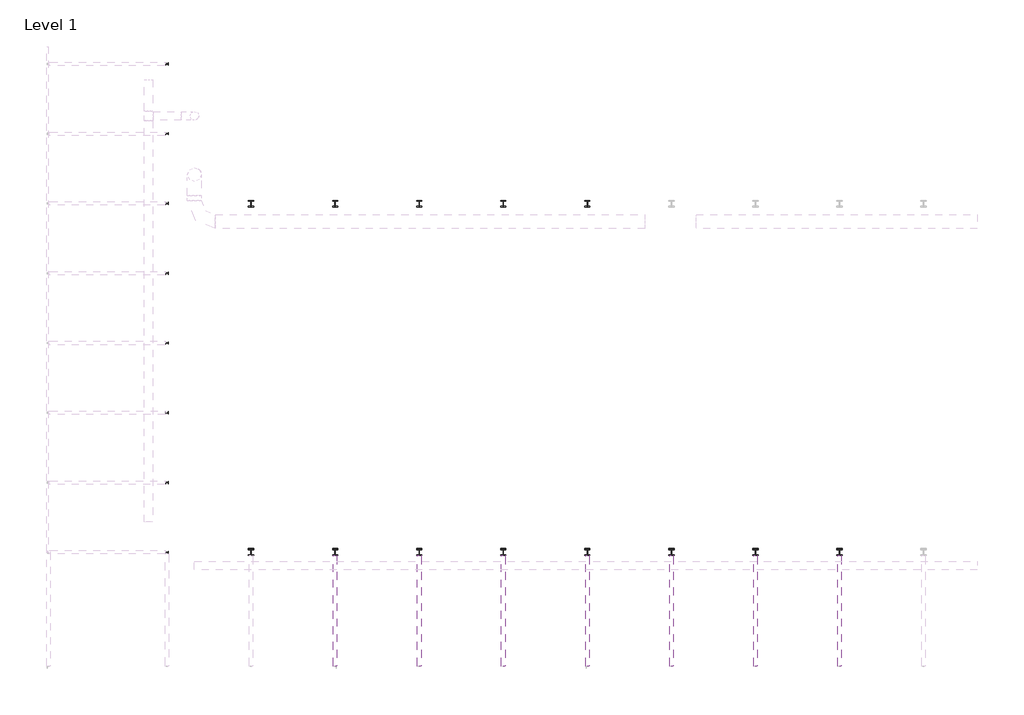
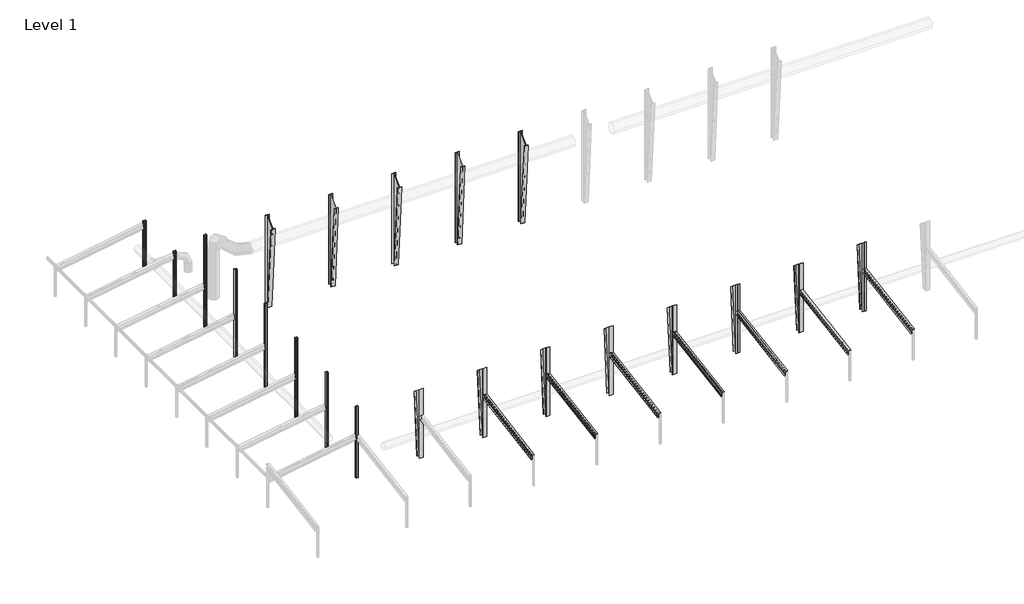
# One storey, part 2 of 3: 21 columns, 7 beams.
"""IFC4 building model written with IfcOpenShell, lengths in millimetres."""

import ifcopenshell
import ifcopenshell.guid

model = None  # the IFC model being written
_history = None  # IfcOwnerHistory: only IFC2X3 demands one
_inside = {}  # id of a spatial element -> (the spatial element, [elements in it])
_under = {}  # id of a project, library or spatial element -> (it, [spatial elements below it])
_declared = {}  # id of a project -> (the project, [libraries it declares])
_typed = {}  # id of a type object -> (the type object, [elements of that type])
_made_of = {}  # id of a material, layer set ... -> (it, [elements and type objects made of it])


def new_model(schema):
    """Start an empty IFC model of exactly this schema.

    Asked for "IFC4X3", IfcOpenShell would pick the latest addendum, in which some entities
    have other attributes; the version numbers below select the first issue.
    IFC2X3 requires an IfcOwnerHistory on every rooted entity: one is made here for all.
    """
    global model, _history
    if schema == "IFC4X3":
        model = ifcopenshell.file(schema_version=(4, 3, 0, 0))
    else:
        model = ifcopenshell.file(schema=schema)
    _inside.clear()
    _under.clear()
    _declared.clear()
    _typed.clear()
    _made_of.clear()
    _history = None
    if model.schema == "IFC2X3":
        org = make("IfcOrganization", Name="unknown")
        user = make(
            "IfcPersonAndOrganization",
            ThePerson=make("IfcPerson", FamilyName="unknown"),
            TheOrganization=org,
        )
        app = make(
            "IfcApplication",
            ApplicationDeveloper=org,
            Version="unknown",
            ApplicationFullName="unknown",
            ApplicationIdentifier="unknown",
        )
        _history = make(
            "IfcOwnerHistory",
            OwningUser=user,
            OwningApplication=app,
            ChangeAction="ADDED",
            CreationDate=0,
        )
    return model


def make(cls, **values):
    """One entity of the class cls with the attributes given. An attribute that is None is left unset."""
    return model.create_entity(
        cls, **{name: value for name, value in values.items() if value is not None}
    )


def rooted(cls, **values):
    """An entity with a GlobalId (a new one), such as an element, a storey or a relation."""
    return make(cls, GlobalId=ifcopenshell.guid.new(), OwnerHistory=_history, **values)


def si_unit(unit_type, name, prefix=None):
    """IfcSIUnit, for example si_unit("LENGTHUNIT", "METRE", prefix="MILLI")."""
    return make("IfcSIUnit", UnitType=unit_type, Prefix=prefix, Name=name)


def assignment(units):
    """IfcUnitAssignment: the units of a project."""
    return None if units is None else make("IfcUnitAssignment", Units=units)


def point(xyz):
    """IfcCartesianPoint."""
    return None if xyz is None else make("IfcCartesianPoint", Coordinates=xyz)


def direction(xyz):
    """IfcDirection."""
    return None if xyz is None else make("IfcDirection", DirectionRatios=xyz)


def frame(location, z_axis=None, x_axis=None):
    """IfcAxis2Placement3D, a coordinate frame: its origin and axes. An axis left out is left unset."""
    return make(
        "IfcAxis2Placement3D",
        Location=point(location),
        Axis=direction(z_axis),
        RefDirection=direction(x_axis),
    )


def frame_2d(location, x_axis=None):
    """IfcAxis2Placement2D, a coordinate frame in the plane: its origin and x axis."""
    return make(
        "IfcAxis2Placement2D", Location=point(location), RefDirection=direction(x_axis)
    )


def origin():
    """The frame at (0, 0, 0) with its axes left unset."""
    return frame((0.0, 0.0, 0.0))


def origin_with_axes():
    """The frame at (0, 0, 0) with the z axis (0, 0, 1) and the x axis (1, 0, 0) written out."""
    return frame((0.0, 0.0, 0.0), z_axis=(0.0, 0.0, 1.0), x_axis=(1.0, 0.0, 0.0))


def place(relative_to, where):
    """IfcLocalPlacement: puts the frame where relative to a parent placement (None: the world)."""
    return make(
        "IfcLocalPlacement", PlacementRelTo=relative_to, RelativePlacement=where
    )


def context(
    kind, dimensions, precision=None, world=None, true_north=None, identifier=None
):
    """IfcGeometricRepresentationContext, for example the 3D "Model" context."""
    return make(
        "IfcGeometricRepresentationContext",
        ContextIdentifier=identifier,
        ContextType=kind,
        CoordinateSpaceDimension=dimensions,
        Precision=precision,
        WorldCoordinateSystem=world,
        TrueNorth=true_north,
    )


def project(units=None, contexts=None):
    """IfcProject with its units and contexts."""
    return rooted(
        "IfcProject",
        Name="project",
        RepresentationContexts=contexts,
        UnitsInContext=assignment(units),
    )


def spatial(cls, under=None, at=None, **own):
    """A site, building, storey or space (cls), placed at a placement, below another one or the project."""
    s = rooted(cls, ObjectPlacement=at, **own)
    if under is not None:
        _under.setdefault(under.id(), (under, []))[1].append(s)
    return s


def polyline(points):
    """IfcPolyline through the points."""
    return make("IfcPolyline", Points=[point(p) for p in points])


def circle_curve(where, radius):
    """IfcCircle in the frame where."""
    return make("IfcCircle", Position=where, Radius=radius)


def trimmed(basis, trim1, trim2, sense, master):
    """IfcTrimmedCurve: the piece of a basis curve between two trims."""
    return make(
        "IfcTrimmedCurve",
        BasisCurve=basis,
        Trim1=trim1,
        Trim2=trim2,
        SenseAgreement=sense,
        MasterRepresentation=master,
    )


def segment(curve, same_sense, transition):
    """IfcCompositeCurveSegment."""
    return make(
        "IfcCompositeCurveSegment",
        Transition=transition,
        SameSense=same_sense,
        ParentCurve=curve,
    )


def composite_curve(segments, self_intersect=None):
    """IfcCompositeCurve: segments joined end to end."""
    return make("IfcCompositeCurve", Segments=segments, SelfIntersect=self_intersect)


def outline(outer, holes=None, kind="AREA"):
    """IfcArbitraryClosedProfileDef: a profile drawn as a closed curve; with holes, ...WithVoids."""
    if holes is None:
        return make("IfcArbitraryClosedProfileDef", ProfileType=kind, OuterCurve=outer)
    return make(
        "IfcArbitraryProfileDefWithVoids",
        ProfileType=kind,
        OuterCurve=outer,
        InnerCurves=holes,
    )


def extrude(swept, where, along, depth):
    """IfcExtrudedAreaSolid: the profile swept, set in the frame where, extruded along a direction by depth."""
    return make(
        "IfcExtrudedAreaSolid",
        SweptArea=swept,
        Position=where,
        ExtrudedDirection=direction(along),
        Depth=depth,
    )


def shape(context_of_items, identifier, shape_type, items):
    """IfcShapeRepresentation: the items that make up one representation, for example the "Body"."""
    return make(
        "IfcShapeRepresentation",
        ContextOfItems=context_of_items,
        RepresentationIdentifier=identifier,
        RepresentationType=shape_type,
        Items=items,
    )


def source(mapping_origin, context_of_items, identifier, shape_type, items):
    """IfcRepresentationMap: a shape defined once, which mapped items show again and again."""
    return make(
        "IfcRepresentationMap",
        MappingOrigin=mapping_origin,
        MappedRepresentation=shape(context_of_items, identifier, shape_type, items),
    )


def transform(
    local_origin,
    x_axis=None,
    y_axis=None,
    z_axis=None,
    scale=None,
    scale2=None,
    scale3=None,
    uniform=True,
):
    """IfcCartesianTransformationOperator3D, or its non-uniform kind. x_axis, y_axis, z_axis: its Axis1, 2, 3."""
    if uniform:
        return make(
            "IfcCartesianTransformationOperator3D",
            Axis1=direction(x_axis),
            Axis2=direction(y_axis),
            LocalOrigin=point(local_origin),
            Scale=scale,
            Axis3=direction(z_axis),
        )
    return make(
        "IfcCartesianTransformationOperator3DnonUniform",
        Axis1=direction(x_axis),
        Axis2=direction(y_axis),
        LocalOrigin=point(local_origin),
        Scale=scale,
        Axis3=direction(z_axis),
        Scale2=scale2,
        Scale3=scale3,
    )


def mapped(mapping_source, mapping_target):
    """IfcMappedItem: shows the shape of a source again, moved by a transform."""
    return make(
        "IfcMappedItem", MappingSource=mapping_source, MappingTarget=mapping_target
    )


def made_of(thing, what):
    """Note that an element or type object is made of a material, layer set ...; save() writes the relation."""
    if what is not None:
        _made_of.setdefault(what.id(), (what, []))[1].append(thing)
    return thing


def element(
    cls,
    number,
    at=None,
    inside=None,
    cuts=None,
    type_object=None,
    material=None,
    context=None,
    identifier="Body",
    shape_type=None,
    held_by="IfcProductDefinitionShape",
    body=None,
    shapes=None,
    **own,
):
    """One element of the class cls, such as IfcWall. Its Tag is "e" and its number.

    at: its placement. inside: the storey or other place that contains it. cuts: it is an
    opening in that element (IfcRelVoidsElement). A single representation is given by context,
    identifier, shape_type and body (its items); several are given by shapes. held_by: the class
    of the entity that holds the representations. save() writes the other relations.
    """
    e = rooted(cls, Tag="e%d" % number, ObjectPlacement=at, **own)
    if body is not None:
        shapes = [shape(context, identifier, shape_type, body)]
    if shapes is not None:
        e.Representation = make(held_by, Representations=shapes)
    if inside is not None:
        _inside.setdefault(inside.id(), (inside, []))[1].append(e)
    if cuts is not None:
        rooted(
            "IfcRelVoidsElement", RelatingBuildingElement=cuts, RelatedOpeningElement=e
        )
    if type_object is not None:
        _typed.setdefault(type_object.id(), (type_object, []))[1].append(e)
    return made_of(e, material)


def aggregate(whole, parts):
    """IfcRelAggregates: a whole, such as a stair, and the parts it consists of."""
    return rooted("IfcRelAggregates", RelatingObject=whole, RelatedObjects=parts)


def save(model, path):
    """Write the relations noted so far, then the file.

    IfcRelAggregates (storeys below a building ...), IfcRelContainedInSpatialStructure (elements
    in a storey), IfcRelDefinesByType, IfcRelAssociatesMaterial and IfcRelDeclares: one each for
    every whole, place, type object, material and project.
    """
    for whole, parts in _under.values():
        aggregate(whole, parts)
    for where, things in _inside.values():
        rooted(
            "IfcRelContainedInSpatialStructure",
            RelatedElements=things,
            RelatingStructure=where,
        )
    for kind, things in _typed.values():
        rooted("IfcRelDefinesByType", RelatedObjects=things, RelatingType=kind)
    for what, things in _made_of.values():
        rooted("IfcRelAssociatesMaterial", RelatedObjects=things, RelatingMaterial=what)
    for by, libraries in _declared.values():
        rooted("IfcRelDeclares", RelatingContext=by, RelatedDefinitions=libraries)
    model.write(path)


def w_wide_flange_w21x166_c1e76bd8(model_context):
    return source(origin(), model_context, "Body", "SweptSolid", [
        extrude(outline(composite_curve([segment(polyline([(157.48, -251.206), (157.48, -285.75), (-157.48, -285.75), (-157.48, -251.206), (-32.131, -251.206)]), True, "CONTINUOUS"), segment(trimmed(circle_curve(frame_2d((-32.131, -228.6)), 22.606), [point((-32.131, -251.206))], [point((-9.525, -228.6))], True, "CARTESIAN"), True, "CONTINUOUS"), segment(polyline([(-9.525, -228.6), (-9.525, 228.6)]), True, "CONTINUOUS"), segment(trimmed(circle_curve(frame_2d((-32.131, 228.6)), 22.606), [point((-9.525, 228.6))], [point((-32.131, 251.206))], True, "CARTESIAN"), True, "CONTINUOUS"), segment(polyline([(-32.131, 251.206), (-157.48, 251.206), (-157.48, 285.75), (157.48, 285.75), (157.48, 251.206), (32.131, 251.206)]), True, "CONTINUOUS"), segment(trimmed(circle_curve(frame_2d((32.131, 228.6)), 22.606), [point((32.131, 251.206))], [point((9.525, 228.6))], True, "CARTESIAN"), True, "CONTINUOUS"), segment(polyline([(9.525, 228.6), (9.525, -228.6)]), True, "CONTINUOUS"), segment(trimmed(circle_curve(frame_2d((32.131, -228.6)), 22.606), [point((9.525, -228.6))], [point((32.131, -251.206))], True, "CARTESIAN"), True, "CONTINUOUS"), segment(polyline([(32.131, -251.206), (157.48, -251.206)]), True, "CONTINUOUS")], self_intersect=False)), frame((-4963.0833359, 0.0, 0.0), z_axis=(1.0, 0.0, 0.0), x_axis=(0.0, 1.0, 0.0)), (0.0, 0.0, 1.0), 9743.826275),
    ])


model = new_model("IFC4")

# Units and contexts
model_context = context("Model", 3, world=origin())
ifc_project = project(units=[si_unit("LENGTHUNIT", "METRE", prefix="MILLI")], contexts=[model_context])

# Site, building, storey
site = spatial("IfcSite", under=ifc_project)
building = spatial("IfcBuilding", under=site)
storey = spatial("IfcBuildingStorey", under=building, Name="Level 1", Elevation=0.0)

# Beams
placement = place(None, origin())
w_wide_flange_w21x166_shape = w_wide_flange_w21x166_c1e76bd8(model_context)
element("IfcBeam", 1, ObjectType="W-Wide Flange : W21X166", at=placement, inside=storey, context=model_context, shape_type="MappedRepresentation", body=[
    mapped(w_wide_flange_w21x166_shape, transform((593709.511724, -572720.5413841, 4206.1084345), x_axis=(0.0, 0.9863939238321447, 0.16439898730535185), y_axis=(-1.0000000000000002, 0.0, 0.0), z_axis=(0.0, -0.16439898730535218, 0.9863939238321446))),
])
element("IfcBeam", 2, ObjectType="W-Wide Flange : W21X166", at=placement, inside=storey, context=model_context, shape_type="MappedRepresentation", body=[
    mapped(w_wide_flange_w21x166_shape, transform((601050.111724, -572720.5413842, 4206.1084345), x_axis=(0.0, 0.9863939238321447, 0.16439898730535185), y_axis=(-1.0000000000000002, 0.0, 0.0), z_axis=(0.0, -0.16439898730535224, 0.9863939238321446))),
])
element("IfcBeam", 3, ObjectType="W-Wide Flange : W21X166", at=placement, inside=storey, context=model_context, shape_type="MappedRepresentation", body=[
    mapped(w_wide_flange_w21x166_shape, transform((608390.7117241, -572720.5413842, 4206.1084345), x_axis=(0.0, 0.9863939238321447, 0.16439898730535185), y_axis=(-1.0000000000000002, 0.0, 0.0), z_axis=(0.0, -0.16439898730535218, 0.9863939238321446))),
])
element("IfcBeam", 4, ObjectType="W-Wide Flange : W21X166", at=placement, inside=storey, context=model_context, shape_type="MappedRepresentation", body=[
    mapped(w_wide_flange_w21x166_shape, transform((615731.3117241, -572720.5413842, 4206.1084345), x_axis=(0.0, 0.9863939238321447, 0.16439898730535185), y_axis=(-1.0, 0.0, 0.0), z_axis=(0.0, -0.16439898730535227, 0.9863939238321445))),
])
element("IfcBeam", 5, ObjectType="W-Wide Flange : W21X166", at=placement, inside=storey, context=model_context, shape_type="MappedRepresentation", body=[
    mapped(w_wide_flange_w21x166_shape, transform((623071.9117241, -572720.5413842, 4206.1084345), x_axis=(0.0, 0.9863939238321447, 0.16439898730535185), y_axis=(-1.0, 0.0, 0.0), z_axis=(0.0, -0.16439898730535227, 0.9863939238321445))),
])
element("IfcBeam", 6, ObjectType="W-Wide Flange : W21X166", at=placement, inside=storey, context=model_context, shape_type="MappedRepresentation", body=[
    mapped(w_wide_flange_w21x166_shape, transform((630412.5117241, -572720.5413842, 4206.1084345), x_axis=(0.0, 0.9863939238321447, 0.16439898730535185), y_axis=(-1.0000000000000002, 0.0, 0.0), z_axis=(0.0, -0.16439898730535218, 0.9863939238321446))),
])
element("IfcBeam", 7, ObjectType="W-Wide Flange : W21X166", at=placement, inside=storey, context=model_context, shape_type="MappedRepresentation", body=[
    mapped(w_wide_flange_w21x166_shape, transform((637753.1117241, -572720.5413843, 4206.1084345), x_axis=(0.0, 0.9863939238321447, 0.16439898730535185), y_axis=(-1.0000000000000002, 0.0, 0.0), z_axis=(0.0, -0.16439898730535224, 0.9863939238321446))),
])

# Columns
element("IfcColumn", 8, ObjectType="Column - Tapered : High", at=placement, inside=storey, context=model_context, shape_type="SweptSolid", body=[
    extrude(outline(polyline([(-536989.0913841, 0.0), (-537433.5204732, 0.0), (-538098.9322262, 9950.5826509), (-536989.0913841, 10985.5259793), (-536989.0913841, 0.0)])), frame((586353.0367239, 0.0, 0.0), z_axis=(1.0, 0.0, 0.0), x_axis=(0.0, 1.0, 0.0)), (0.0, 0.0, 1.0), 31.75),
    extrude(outline(polyline([(-536957.3413841, 11015.1333333), (-536957.3413841, 0.0), (-536989.0913841, 0.0), (-536989.0913841, 10985.5259793), (-536957.3413841, 11015.1333333)])), frame((586140.3117239, 0.0, 0.0), z_axis=(1.0, 0.0, 0.0), x_axis=(0.0, 1.0, 0.0)), (0.0, 0.0, 1.0), 457.2),
    extrude(outline(polyline([(-537433.5204732, 0.0), (-537465.3413841, 0.0), (-538128.8852991, 9922.6509585), (-538098.9322262, 9950.5826509), (-537433.5204732, 0.0)])), frame((586140.3117239, 0.0, 0.0), z_axis=(1.0, 0.0, 0.0), x_axis=(0.0, 1.0, 0.0)), (0.0, 0.0, 1.0), 457.2),
])
element("IfcColumn", 9, ObjectType="Column - Tapered : High", at=placement, inside=storey, context=model_context, shape_type="SweptSolid", body=[
    extrude(outline(polyline([(-536989.0913841, 0.0), (-537433.5204732, 0.0), (-538098.9322262, 9950.5826509), (-536989.0913841, 10985.5259793), (-536989.0913841, 0.0)])), frame((593693.6367239, 0.0, 0.0), z_axis=(1.0, 0.0, 0.0), x_axis=(0.0, 1.0, 0.0)), (0.0, 0.0, 1.0), 31.75),
    extrude(outline(polyline([(-536957.3413841, 11015.1333333), (-536957.3413841, 0.0), (-536989.0913841, 0.0), (-536989.0913841, 10985.5259793), (-536957.3413841, 11015.1333333)])), frame((593480.9117239, 0.0, 0.0), z_axis=(1.0, 0.0, 0.0), x_axis=(0.0, 1.0, 0.0)), (0.0, 0.0, 1.0), 457.2),
    extrude(outline(polyline([(-537433.5204732, 0.0), (-537465.3413841, 0.0), (-538128.8852991, 9922.6509585), (-538098.9322262, 9950.5826509), (-537433.5204732, 0.0)])), frame((593480.9117239, 0.0, 0.0), z_axis=(1.0, 0.0, 0.0), x_axis=(0.0, 1.0, 0.0)), (0.0, 0.0, 1.0), 457.2),
])
element("IfcColumn", 10, ObjectType="Column - Tapered : High", at=placement, inside=storey, context=model_context, shape_type="SweptSolid", body=[
    extrude(outline(polyline([(-536989.0913841, 0.0), (-537433.5204732, 0.0), (-538098.9322262, 9950.5826509), (-536989.0913841, 10985.5259793), (-536989.0913841, 0.0)])), frame((601034.2367239, 0.0, 0.0), z_axis=(1.0, 0.0, 0.0), x_axis=(0.0, 1.0, 0.0)), (0.0, 0.0, 1.0), 31.75),
    extrude(outline(polyline([(-536957.3413841, 11015.1333333), (-536957.3413841, 0.0), (-536989.0913841, 0.0), (-536989.0913841, 10985.5259793), (-536957.3413841, 11015.1333333)])), frame((600821.5117239, 0.0, 0.0), z_axis=(1.0, 0.0, 0.0), x_axis=(0.0, 1.0, 0.0)), (0.0, 0.0, 1.0), 457.2),
    extrude(outline(polyline([(-537433.5204732, 0.0), (-537465.3413841, 0.0), (-538128.8852991, 9922.6509585), (-538098.9322262, 9950.5826509), (-537433.5204732, 0.0)])), frame((600821.5117239, 0.0, 0.0), z_axis=(1.0, 0.0, 0.0), x_axis=(0.0, 1.0, 0.0)), (0.0, 0.0, 1.0), 457.2),
])
element("IfcColumn", 11, ObjectType="Column - Tapered : High", at=placement, inside=storey, context=model_context, shape_type="SweptSolid", body=[
    extrude(outline(polyline([(-536989.0913841, 0.0), (-537433.5204732, 0.0), (-538098.9322262, 9950.5826509), (-536989.0913841, 10985.5259793), (-536989.0913841, 0.0)])), frame((608374.8367239, 0.0, 0.0), z_axis=(1.0, 0.0, 0.0), x_axis=(0.0, 1.0, 0.0)), (0.0, 0.0, 1.0), 31.75),
    extrude(outline(polyline([(-536957.3413841, 11015.1333333), (-536957.3413841, 0.0), (-536989.0913841, 0.0), (-536989.0913841, 10985.5259793), (-536957.3413841, 11015.1333333)])), frame((608162.1117239, 0.0, 0.0), z_axis=(1.0, 0.0, 0.0), x_axis=(0.0, 1.0, 0.0)), (0.0, 0.0, 1.0), 457.2),
    extrude(outline(polyline([(-537433.5204732, 0.0), (-537465.3413841, 0.0), (-538128.8852991, 9922.6509585), (-538098.9322262, 9950.5826509), (-537433.5204732, 0.0)])), frame((608162.1117239, 0.0, 0.0), z_axis=(1.0, 0.0, 0.0), x_axis=(0.0, 1.0, 0.0)), (0.0, 0.0, 1.0), 457.2),
])
element("IfcColumn", 12, ObjectType="Column - Tapered : High", at=placement, inside=storey, context=model_context, shape_type="SweptSolid", body=[
    extrude(outline(polyline([(-536989.0913841, 0.0), (-537433.5204732, 0.0), (-538098.9322262, 9950.5826509), (-536989.0913841, 10985.5259793), (-536989.0913841, 0.0)])), frame((615715.4367239, 0.0, 0.0), z_axis=(1.0, 0.0, 0.0), x_axis=(0.0, 1.0, 0.0)), (0.0, 0.0, 1.0), 31.75),
    extrude(outline(polyline([(-536957.3413841, 11015.1333333), (-536957.3413841, 0.0), (-536989.0913841, 0.0), (-536989.0913841, 10985.5259793), (-536957.3413841, 11015.1333333)])), frame((615502.7117239, 0.0, 0.0), z_axis=(1.0, 0.0, 0.0), x_axis=(0.0, 1.0, 0.0)), (0.0, 0.0, 1.0), 457.2),
    extrude(outline(polyline([(-537433.5204732, 0.0), (-537465.3413841, 0.0), (-538128.8852991, 9922.6509585), (-538098.9322262, 9950.5826509), (-537433.5204732, 0.0)])), frame((615502.7117239, 0.0, 0.0), z_axis=(1.0, 0.0, 0.0), x_axis=(0.0, 1.0, 0.0)), (0.0, 0.0, 1.0), 457.2),
])
element("IfcColumn", 13, ObjectType="Column - Tapered : Low", at=placement, inside=storey, context=model_context, shape_type="SweptSolid", body=[
    extrude(outline(polyline([(-567913.5913841, 0.0), (-567913.5913841, 8407.0893569), (-566919.6186142, 7602.1860785), (-567469.1742343, 0.0), (-567913.5913841, 0.0)])), frame((586353.0367239, 0.0, 0.0), z_axis=(1.0, 0.0, 0.0), x_axis=(0.0, 1.0, 0.0)), (0.0, 0.0, 1.0), 31.75),
    extrude(outline(polyline([(-567945.3413841, 8432.8), (-567913.5913841, 8407.0893569), (-567913.5913841, 0.0), (-567945.3413841, 0.0), (-567945.3413841, 8432.8)])), frame((586140.3117239, 0.0, 0.0), z_axis=(1.0, 0.0, 0.0), x_axis=(0.0, 1.0, 0.0)), (0.0, 0.0, 1.0), 457.2),
    extrude(outline(polyline([(-567469.1742343, 0.0), (-566919.6186142, 7602.1860785), (-566889.5461633, 7577.8338879), (-567437.3413841, 0.0), (-567469.1742343, 0.0)])), frame((586140.3117239, 0.0, 0.0), z_axis=(1.0, 0.0, 0.0), x_axis=(0.0, 1.0, 0.0)), (0.0, 0.0, 1.0), 457.2),
])
element("IfcColumn", 14, ObjectType="Column - Tapered : Low", at=placement, inside=storey, context=model_context, shape_type="SweptSolid", body=[
    extrude(outline(polyline([(-567913.5913841, 0.0), (-567913.5913841, 8407.0893569), (-566919.6186142, 7602.1860785), (-567469.1742343, 0.0), (-567913.5913841, 0.0)])), frame((593693.6367239, 0.0, 0.0), z_axis=(1.0, 0.0, 0.0), x_axis=(0.0, 1.0, 0.0)), (0.0, 0.0, 1.0), 31.75),
    extrude(outline(polyline([(-567945.3413841, 8432.8), (-567913.5913841, 8407.0893569), (-567913.5913841, 0.0), (-567945.3413841, 0.0), (-567945.3413841, 8432.8)])), frame((593480.9117239, 0.0, 0.0), z_axis=(1.0, 0.0, 0.0), x_axis=(0.0, 1.0, 0.0)), (0.0, 0.0, 1.0), 457.2),
    extrude(outline(polyline([(-567469.1742343, 0.0), (-566919.6186142, 7602.1860785), (-566889.5461633, 7577.8338879), (-567437.3413841, 0.0), (-567469.1742343, 0.0)])), frame((593480.9117239, 0.0, 0.0), z_axis=(1.0, 0.0, 0.0), x_axis=(0.0, 1.0, 0.0)), (0.0, 0.0, 1.0), 457.2),
])
element("IfcColumn", 15, ObjectType="Column - Tapered : Low", at=placement, inside=storey, context=model_context, shape_type="SweptSolid", body=[
    extrude(outline(polyline([(-567913.5913841, 0.0), (-567913.5913841, 8407.0893569), (-566919.6186142, 7602.1860785), (-567469.1742343, 0.0), (-567913.5913841, 0.0)])), frame((601034.2367239, 0.0, 0.0), z_axis=(1.0, 0.0, 0.0), x_axis=(0.0, 1.0, 0.0)), (0.0, 0.0, 1.0), 31.75),
    extrude(outline(polyline([(-567945.3413841, 8432.8), (-567913.5913841, 8407.0893569), (-567913.5913841, 0.0), (-567945.3413841, 0.0), (-567945.3413841, 8432.8)])), frame((600821.5117239, 0.0, 0.0), z_axis=(1.0, 0.0, 0.0), x_axis=(0.0, 1.0, 0.0)), (0.0, 0.0, 1.0), 457.2),
    extrude(outline(polyline([(-567469.1742343, 0.0), (-566919.6186142, 7602.1860785), (-566889.5461633, 7577.8338879), (-567437.3413841, 0.0), (-567469.1742343, 0.0)])), frame((600821.5117239, 0.0, 0.0), z_axis=(1.0, 0.0, 0.0), x_axis=(0.0, 1.0, 0.0)), (0.0, 0.0, 1.0), 457.2),
])
element("IfcColumn", 16, ObjectType="Column - Tapered : Low", at=placement, inside=storey, context=model_context, shape_type="SweptSolid", body=[
    extrude(outline(polyline([(-567913.5913841, 0.0), (-567913.5913841, 8407.0893569), (-566919.6186142, 7602.1860785), (-567469.1742343, 0.0), (-567913.5913841, 0.0)])), frame((608374.8367239, 0.0, 0.0), z_axis=(1.0, 0.0, 0.0), x_axis=(0.0, 1.0, 0.0)), (0.0, 0.0, 1.0), 31.75),
    extrude(outline(polyline([(-567945.3413841, 8432.8), (-567913.5913841, 8407.0893569), (-567913.5913841, 0.0), (-567945.3413841, 0.0), (-567945.3413841, 8432.8)])), frame((608162.1117239, 0.0, 0.0), z_axis=(1.0, 0.0, 0.0), x_axis=(0.0, 1.0, 0.0)), (0.0, 0.0, 1.0), 457.2),
    extrude(outline(polyline([(-567469.1742343, 0.0), (-566919.6186142, 7602.1860785), (-566889.5461633, 7577.8338879), (-567437.3413841, 0.0), (-567469.1742343, 0.0)])), frame((608162.1117239, 0.0, 0.0), z_axis=(1.0, 0.0, 0.0), x_axis=(0.0, 1.0, 0.0)), (0.0, 0.0, 1.0), 457.2),
])
element("IfcColumn", 17, ObjectType="Column - Tapered : Low", at=placement, inside=storey, context=model_context, shape_type="SweptSolid", body=[
    extrude(outline(polyline([(-567913.5913841, 0.0), (-567913.5913841, 8407.0893569), (-566919.6186142, 7602.1860785), (-567469.1742343, 0.0), (-567913.5913841, 0.0)])), frame((615715.4367239, 0.0, 0.0), z_axis=(1.0, 0.0, 0.0), x_axis=(0.0, 1.0, 0.0)), (0.0, 0.0, 1.0), 31.75),
    extrude(outline(polyline([(-567945.3413841, 8432.8), (-567913.5913841, 8407.0893569), (-567913.5913841, 0.0), (-567945.3413841, 0.0), (-567945.3413841, 8432.8)])), frame((615502.7117239, 0.0, 0.0), z_axis=(1.0, 0.0, 0.0), x_axis=(0.0, 1.0, 0.0)), (0.0, 0.0, 1.0), 457.2),
    extrude(outline(polyline([(-567469.1742343, 0.0), (-566919.6186142, 7602.1860785), (-566889.5461633, 7577.8338879), (-567437.3413841, 0.0), (-567469.1742343, 0.0)])), frame((615502.7117239, 0.0, 0.0), z_axis=(1.0, 0.0, 0.0), x_axis=(0.0, 1.0, 0.0)), (0.0, 0.0, 1.0), 457.2),
])
element("IfcColumn", 18, ObjectType="Column - Tapered : Low", at=placement, inside=storey, context=model_context, shape_type="SweptSolid", body=[
    extrude(outline(polyline([(-567913.5913841, 0.0), (-567913.5913841, 8407.0893569), (-566919.6186142, 7602.1860785), (-567469.1742343, 0.0), (-567913.5913841, 0.0)])), frame((623056.0367239, 0.0, 0.0), z_axis=(1.0, 0.0, 0.0), x_axis=(0.0, 1.0, 0.0)), (0.0, 0.0, 1.0), 31.75),
    extrude(outline(polyline([(-567945.3413841, 8432.8), (-567913.5913841, 8407.0893569), (-567913.5913841, 0.0), (-567945.3413841, 0.0), (-567945.3413841, 8432.8)])), frame((622843.3117239, 0.0, 0.0), z_axis=(1.0, 0.0, 0.0), x_axis=(0.0, 1.0, 0.0)), (0.0, 0.0, 1.0), 457.2),
    extrude(outline(polyline([(-567469.1742343, 0.0), (-566919.6186142, 7602.1860785), (-566889.5461633, 7577.8338879), (-567437.3413841, 0.0), (-567469.1742343, 0.0)])), frame((622843.3117239, 0.0, 0.0), z_axis=(1.0, 0.0, 0.0), x_axis=(0.0, 1.0, 0.0)), (0.0, 0.0, 1.0), 457.2),
])
element("IfcColumn", 19, ObjectType="Column - Tapered : Low", at=placement, inside=storey, context=model_context, shape_type="SweptSolid", body=[
    extrude(outline(polyline([(-567913.5913841, 0.0), (-567913.5913841, 8407.0893569), (-566919.6186142, 7602.1860785), (-567469.1742343, 0.0), (-567913.5913841, 0.0)])), frame((630396.6367239, 0.0, 0.0), z_axis=(1.0, 0.0, 0.0), x_axis=(0.0, 1.0, 0.0)), (0.0, 0.0, 1.0), 31.75),
    extrude(outline(polyline([(-567945.3413841, 8432.8), (-567913.5913841, 8407.0893569), (-567913.5913841, 0.0), (-567945.3413841, 0.0), (-567945.3413841, 8432.8)])), frame((630183.9117239, 0.0, 0.0), z_axis=(1.0, 0.0, 0.0), x_axis=(0.0, 1.0, 0.0)), (0.0, 0.0, 1.0), 457.2),
    extrude(outline(polyline([(-567469.1742343, 0.0), (-566919.6186142, 7602.1860785), (-566889.5461633, 7577.8338879), (-567437.3413841, 0.0), (-567469.1742343, 0.0)])), frame((630183.9117239, 0.0, 0.0), z_axis=(1.0, 0.0, 0.0), x_axis=(0.0, 1.0, 0.0)), (0.0, 0.0, 1.0), 457.2),
])
element("IfcColumn", 20, ObjectType="Column - Tapered : Low", at=placement, inside=storey, context=model_context, shape_type="SweptSolid", body=[
    extrude(outline(polyline([(-567913.5913841, 0.0), (-567913.5913841, 8407.0893569), (-566919.6186142, 7602.1860785), (-567469.1742343, 0.0), (-567913.5913841, 0.0)])), frame((637737.2367239, 0.0, 0.0), z_axis=(1.0, 0.0, 0.0), x_axis=(0.0, 1.0, 0.0)), (0.0, 0.0, 1.0), 31.75),
    extrude(outline(polyline([(-567945.3413841, 8432.8), (-567913.5913841, 8407.0893569), (-567913.5913841, 0.0), (-567945.3413841, 0.0), (-567945.3413841, 8432.8)])), frame((637524.5117239, 0.0, 0.0), z_axis=(1.0, 0.0, 0.0), x_axis=(0.0, 1.0, 0.0)), (0.0, 0.0, 1.0), 457.2),
    extrude(outline(polyline([(-567469.1742343, 0.0), (-566919.6186142, 7602.1860785), (-566889.5461633, 7577.8338879), (-567437.3413841, 0.0), (-567469.1742343, 0.0)])), frame((637524.5117239, 0.0, 0.0), z_axis=(1.0, 0.0, 0.0), x_axis=(0.0, 1.0, 0.0)), (0.0, 0.0, 1.0), 457.2),
])
element("IfcColumn", 21, ObjectType="W-Wide Flange-Column : W10X33", at=placement, inside=storey, context=model_context, shape_type="SweptSolid", body=[
    extrude(outline(composite_curve([segment(polyline([(579151.8886771, -537312.4452903), (579140.8753958, -537312.4452903), (579140.8753958, -537232.5741966)]), True, "CONTINUOUS"), segment(trimmed(circle_curve(frame_2d((579123.3136771, -537232.5741966)), 17.5617188), [point((579140.8753958, -537232.5741966))], [point((579123.3136771, -537215.0124778))], True, "CARTESIAN"), True, "CONTINUOUS"), segment(polyline([(579123.3136771, -537215.0124778), (578933.3097708, -537215.0124778)]), True, "CONTINUOUS"), segment(trimmed(circle_curve(frame_2d((578933.3097708, -537232.5741966)), 17.5617188), [point((578933.3097708, -537215.0124778))], [point((578915.7480521, -537232.5741966))], True, "CARTESIAN"), True, "CONTINUOUS"), segment(polyline([(578915.7480521, -537232.5741966), (578915.7480521, -537312.4452903), (578904.7347708, -537312.4452903), (578904.7347708, -537110.2374778), (578915.7480521, -537110.2374778), (578915.7480521, -537190.1085716)]), True, "CONTINUOUS"), segment(trimmed(circle_curve(frame_2d((578933.3097708, -537190.1085716)), 17.5617187), [point((578915.7480521, -537190.1085716))], [point((578933.3097708, -537207.6702903))], True, "CARTESIAN"), True, "CONTINUOUS"), segment(polyline([(578933.3097708, -537207.6702903), (579123.3136771, -537207.6702903)]), True, "CONTINUOUS"), segment(trimmed(circle_curve(frame_2d((579123.3136771, -537190.1085716)), 17.5617187), [point((579123.3136771, -537207.6702903))], [point((579140.8753958, -537190.1085716))], True, "CARTESIAN"), True, "CONTINUOUS"), segment(polyline([(579140.8753958, -537190.1085716), (579140.8753958, -537110.2374778), (579151.8886771, -537110.2374778), (579151.8886771, -537312.4452903)]), True, "CONTINUOUS")], self_intersect=False)), origin_with_axes(), (0.0, 0.0, 1.0), 11291.2217597),
])
element("IfcColumn", 22, ObjectType="W-Wide Flange-Column : W10X33", at=placement, inside=storey, context=model_context, shape_type="SweptSolid", body=[
    extrude(outline(composite_curve([segment(polyline([(579151.8886771, -567792.4452903), (579140.8753958, -567792.4452903), (579140.8753958, -567712.5741966)]), True, "CONTINUOUS"), segment(trimmed(circle_curve(frame_2d((579123.3136771, -567712.5741966)), 17.5617188), [point((579140.8753958, -567712.5741966))], [point((579123.3136771, -567695.0124778))], True, "CARTESIAN"), True, "CONTINUOUS"), segment(polyline([(579123.3136771, -567695.0124778), (578933.3097708, -567695.0124778)]), True, "CONTINUOUS"), segment(trimmed(circle_curve(frame_2d((578933.3097708, -567712.5741966)), 17.5617188), [point((578933.3097708, -567695.0124778))], [point((578915.7480521, -567712.5741966))], True, "CARTESIAN"), True, "CONTINUOUS"), segment(polyline([(578915.7480521, -567712.5741966), (578915.7480521, -567792.4452903), (578904.7347708, -567792.4452903), (578904.7347708, -567590.2374778), (578915.7480521, -567590.2374778), (578915.7480521, -567670.1085716)]), True, "CONTINUOUS"), segment(trimmed(circle_curve(frame_2d((578933.3097708, -567670.1085716)), 17.5617187), [point((578915.7480521, -567670.1085716))], [point((578933.3097708, -567687.6702903))], True, "CARTESIAN"), True, "CONTINUOUS"), segment(polyline([(578933.3097708, -567687.6702903), (579123.3136771, -567687.6702903)]), True, "CONTINUOUS"), segment(trimmed(circle_curve(frame_2d((579123.3136771, -567670.1085716)), 17.5617187), [point((579123.3136771, -567687.6702903))], [point((579140.8753958, -567670.1085716))], True, "CARTESIAN"), True, "CONTINUOUS"), segment(polyline([(579140.8753958, -567670.1085716), (579140.8753958, -567590.2374778), (579151.8886771, -567590.2374778), (579151.8886771, -567792.4452903)]), True, "CONTINUOUS")], self_intersect=False)), origin_with_axes(), (0.0, 0.0, 1.0), 8751.2217597),
])
element("IfcColumn", 23, ObjectType="W-Wide Flange-Column : W10X33", at=placement, inside=storey, context=model_context, shape_type="SweptSolid", body=[
    extrude(outline(composite_curve([segment(polyline([(579151.8886771, -525120.4452903), (579140.8753958, -525120.4452903), (579140.8753958, -525040.5741966)]), True, "CONTINUOUS"), segment(trimmed(circle_curve(frame_2d((579123.3136771, -525040.5741966)), 17.5617188), [point((579140.8753958, -525040.5741966))], [point((579123.3136771, -525023.0124778))], True, "CARTESIAN"), True, "CONTINUOUS"), segment(polyline([(579123.3136771, -525023.0124778), (578933.3097708, -525023.0124778)]), True, "CONTINUOUS"), segment(trimmed(circle_curve(frame_2d((578933.3097708, -525040.5741966)), 17.5617188), [point((578933.3097708, -525023.0124778))], [point((578915.7480521, -525040.5741966))], True, "CARTESIAN"), True, "CONTINUOUS"), segment(polyline([(578915.7480521, -525040.5741966), (578915.7480521, -525120.4452903), (578904.7347708, -525120.4452903), (578904.7347708, -524918.2374778), (578915.7480521, -524918.2374778), (578915.7480521, -524998.1085716)]), True, "CONTINUOUS"), segment(trimmed(circle_curve(frame_2d((578933.3097708, -524998.1085716)), 17.5617187), [point((578915.7480521, -524998.1085716))], [point((578933.3097708, -525015.6702903))], True, "CARTESIAN"), True, "CONTINUOUS"), segment(polyline([(578933.3097708, -525015.6702903), (579123.3136771, -525015.6702903)]), True, "CONTINUOUS"), segment(trimmed(circle_curve(frame_2d((579123.3136771, -524998.1085716)), 17.5617187), [point((579123.3136771, -525015.6702903))], [point((579140.8753958, -524998.1085716))], True, "CARTESIAN"), True, "CONTINUOUS"), segment(polyline([(579140.8753958, -524998.1085716), (579140.8753958, -524918.2374778), (579151.8886771, -524918.2374778), (579151.8886771, -525120.4452903)]), True, "CONTINUOUS")], self_intersect=False)), origin_with_axes(), (0.0, 0.0, 1.0), 5621.7074549),
])
element("IfcColumn", 24, ObjectType="W-Wide Flange-Column : W10X33", at=placement, inside=storey, context=model_context, shape_type="SweptSolid", body=[
    extrude(outline(composite_curve([segment(polyline([(579151.8886771, -543408.4452903), (579140.8753958, -543408.4452903), (579140.8753958, -543328.5741966)]), True, "CONTINUOUS"), segment(trimmed(circle_curve(frame_2d((579123.3136771, -543328.5741966)), 17.5617188), [point((579140.8753958, -543328.5741966))], [point((579123.3136771, -543311.0124778))], True, "CARTESIAN"), True, "CONTINUOUS"), segment(polyline([(579123.3136771, -543311.0124778), (578933.3097708, -543311.0124778)]), True, "CONTINUOUS"), segment(trimmed(circle_curve(frame_2d((578933.3097708, -543328.5741966)), 17.5617188), [point((578933.3097708, -543311.0124778))], [point((578915.7480521, -543328.5741966))], True, "CARTESIAN"), True, "CONTINUOUS"), segment(polyline([(578915.7480521, -543328.5741966), (578915.7480521, -543408.4452903), (578904.7347708, -543408.4452903), (578904.7347708, -543206.2374778), (578915.7480521, -543206.2374778), (578915.7480521, -543286.1085716)]), True, "CONTINUOUS"), segment(trimmed(circle_curve(frame_2d((578933.3097708, -543286.1085716)), 17.5617187), [point((578915.7480521, -543286.1085716))], [point((578933.3097708, -543303.6702903))], True, "CARTESIAN"), True, "CONTINUOUS"), segment(polyline([(578933.3097708, -543303.6702903), (579123.3136771, -543303.6702903)]), True, "CONTINUOUS"), segment(trimmed(circle_curve(frame_2d((579123.3136771, -543286.1085716)), 17.5617187), [point((579123.3136771, -543303.6702903))], [point((579140.8753958, -543286.1085716))], True, "CARTESIAN"), True, "CONTINUOUS"), segment(polyline([(579140.8753958, -543286.1085716), (579140.8753958, -543206.2374778), (579151.8886771, -543206.2374778), (579151.8886771, -543408.4452903)]), True, "CONTINUOUS")], self_intersect=False)), origin_with_axes(), (0.0, 0.0, 1.0), 10783.2217597),
])
element("IfcColumn", 25, ObjectType="W-Wide Flange-Column : W10X33", at=placement, inside=storey, context=model_context, shape_type="SweptSolid", body=[
    extrude(outline(composite_curve([segment(polyline([(579151.8886771, -549504.4452903), (579140.8753958, -549504.4452903), (579140.8753958, -549424.5741966)]), True, "CONTINUOUS"), segment(trimmed(circle_curve(frame_2d((579123.3136771, -549424.5741966)), 17.5617188), [point((579140.8753958, -549424.5741966))], [point((579123.3136771, -549407.0124778))], True, "CARTESIAN"), True, "CONTINUOUS"), segment(polyline([(579123.3136771, -549407.0124778), (578933.3097708, -549407.0124778)]), True, "CONTINUOUS"), segment(trimmed(circle_curve(frame_2d((578933.3097708, -549424.5741966)), 17.5617188), [point((578933.3097708, -549407.0124778))], [point((578915.7480521, -549424.5741966))], True, "CARTESIAN"), True, "CONTINUOUS"), segment(polyline([(578915.7480521, -549424.5741966), (578915.7480521, -549504.4452903), (578904.7347708, -549504.4452903), (578904.7347708, -549302.2374778), (578915.7480521, -549302.2374778), (578915.7480521, -549382.1085716)]), True, "CONTINUOUS"), segment(trimmed(circle_curve(frame_2d((578933.3097708, -549382.1085716)), 17.5617187), [point((578915.7480521, -549382.1085716))], [point((578933.3097708, -549399.6702903))], True, "CARTESIAN"), True, "CONTINUOUS"), segment(polyline([(578933.3097708, -549399.6702903), (579123.3136771, -549399.6702903)]), True, "CONTINUOUS"), segment(trimmed(circle_curve(frame_2d((579123.3136771, -549382.1085716)), 17.5617187), [point((579123.3136771, -549399.6702903))], [point((579140.8753958, -549382.1085716))], True, "CARTESIAN"), True, "CONTINUOUS"), segment(polyline([(579140.8753958, -549382.1085716), (579140.8753958, -549302.2374778), (579151.8886771, -549302.2374778), (579151.8886771, -549504.4452903)]), True, "CONTINUOUS")], self_intersect=False)), origin_with_axes(), (0.0, 0.0, 1.0), 10275.2217597),
])
element("IfcColumn", 26, ObjectType="W-Wide Flange-Column : W10X33", at=placement, inside=storey, context=model_context, shape_type="SweptSolid", body=[
    extrude(outline(composite_curve([segment(polyline([(579151.8886771, -555600.4452903), (579140.8753958, -555600.4452903), (579140.8753958, -555520.5741966)]), True, "CONTINUOUS"), segment(trimmed(circle_curve(frame_2d((579123.3136771, -555520.5741966)), 17.5617188), [point((579140.8753958, -555520.5741966))], [point((579123.3136771, -555503.0124778))], True, "CARTESIAN"), True, "CONTINUOUS"), segment(polyline([(579123.3136771, -555503.0124778), (578933.3097708, -555503.0124778)]), True, "CONTINUOUS"), segment(trimmed(circle_curve(frame_2d((578933.3097708, -555520.5741966)), 17.5617188), [point((578933.3097708, -555503.0124778))], [point((578915.7480521, -555520.5741966))], True, "CARTESIAN"), True, "CONTINUOUS"), segment(polyline([(578915.7480521, -555520.5741966), (578915.7480521, -555600.4452903), (578904.7347708, -555600.4452903), (578904.7347708, -555398.2374778), (578915.7480521, -555398.2374778), (578915.7480521, -555478.1085716)]), True, "CONTINUOUS"), segment(trimmed(circle_curve(frame_2d((578933.3097708, -555478.1085716)), 17.5617187), [point((578915.7480521, -555478.1085716))], [point((578933.3097708, -555495.6702903))], True, "CARTESIAN"), True, "CONTINUOUS"), segment(polyline([(578933.3097708, -555495.6702903), (579123.3136771, -555495.6702903)]), True, "CONTINUOUS"), segment(trimmed(circle_curve(frame_2d((579123.3136771, -555478.1085716)), 17.5617187), [point((579123.3136771, -555495.6702903))], [point((579140.8753958, -555478.1085716))], True, "CARTESIAN"), True, "CONTINUOUS"), segment(polyline([(579140.8753958, -555478.1085716), (579140.8753958, -555398.2374778), (579151.8886771, -555398.2374778), (579151.8886771, -555600.4452903)]), True, "CONTINUOUS")], self_intersect=False)), origin_with_axes(), (0.0, 0.0, 1.0), 9767.2217597),
])
element("IfcColumn", 27, ObjectType="W-Wide Flange-Column : W10X33", at=placement, inside=storey, context=model_context, shape_type="SweptSolid", body=[
    extrude(outline(composite_curve([segment(polyline([(579151.8886771, -561696.4452903), (579140.8753958, -561696.4452903), (579140.8753958, -561616.5741966)]), True, "CONTINUOUS"), segment(trimmed(circle_curve(frame_2d((579123.3136771, -561616.5741966)), 17.5617188), [point((579140.8753958, -561616.5741966))], [point((579123.3136771, -561599.0124778))], True, "CARTESIAN"), True, "CONTINUOUS"), segment(polyline([(579123.3136771, -561599.0124778), (578933.3097708, -561599.0124778)]), True, "CONTINUOUS"), segment(trimmed(circle_curve(frame_2d((578933.3097708, -561616.5741966)), 17.5617188), [point((578933.3097708, -561599.0124778))], [point((578915.7480521, -561616.5741966))], True, "CARTESIAN"), True, "CONTINUOUS"), segment(polyline([(578915.7480521, -561616.5741966), (578915.7480521, -561696.4452903), (578904.7347708, -561696.4452903), (578904.7347708, -561494.2374778), (578915.7480521, -561494.2374778), (578915.7480521, -561574.1085716)]), True, "CONTINUOUS"), segment(trimmed(circle_curve(frame_2d((578933.3097708, -561574.1085716)), 17.5617187), [point((578915.7480521, -561574.1085716))], [point((578933.3097708, -561591.6702903))], True, "CARTESIAN"), True, "CONTINUOUS"), segment(polyline([(578933.3097708, -561591.6702903), (579123.3136771, -561591.6702903)]), True, "CONTINUOUS"), segment(trimmed(circle_curve(frame_2d((579123.3136771, -561574.1085716)), 17.5617187), [point((579123.3136771, -561591.6702903))], [point((579140.8753958, -561574.1085716))], True, "CARTESIAN"), True, "CONTINUOUS"), segment(polyline([(579140.8753958, -561574.1085716), (579140.8753958, -561494.2374778), (579151.8886771, -561494.2374778), (579151.8886771, -561696.4452903)]), True, "CONTINUOUS")], self_intersect=False)), origin_with_axes(), (0.0, 0.0, 1.0), 9259.2217597),
])
element("IfcColumn", 28, ObjectType="W-Wide Flange-Column : W10X33", at=placement, inside=storey, context=model_context, shape_type="SweptSolid", body=[
    extrude(outline(composite_curve([segment(polyline([(579151.8886771, -531216.4452903), (579140.8753958, -531216.4452903), (579140.8753958, -531136.5741966)]), True, "CONTINUOUS"), segment(trimmed(circle_curve(frame_2d((579123.3136771, -531136.5741966)), 17.5617188), [point((579140.8753958, -531136.5741966))], [point((579123.3136771, -531119.0124778))], True, "CARTESIAN"), True, "CONTINUOUS"), segment(polyline([(579123.3136771, -531119.0124778), (578933.3097708, -531119.0124778)]), True, "CONTINUOUS"), segment(trimmed(circle_curve(frame_2d((578933.3097708, -531136.5741966)), 17.5617188), [point((578933.3097708, -531119.0124778))], [point((578915.7480521, -531136.5741966))], True, "CARTESIAN"), True, "CONTINUOUS"), segment(polyline([(578915.7480521, -531136.5741966), (578915.7480521, -531216.4452903), (578904.7347708, -531216.4452903), (578904.7347708, -531014.2374778), (578915.7480521, -531014.2374778), (578915.7480521, -531094.1085716)]), True, "CONTINUOUS"), segment(trimmed(circle_curve(frame_2d((578933.3097708, -531094.1085716)), 17.5617187), [point((578915.7480521, -531094.1085716))], [point((578933.3097708, -531111.6702903))], True, "CARTESIAN"), True, "CONTINUOUS"), segment(polyline([(578933.3097708, -531111.6702903), (579123.3136771, -531111.6702903)]), True, "CONTINUOUS"), segment(trimmed(circle_curve(frame_2d((579123.3136771, -531094.1085716)), 17.5617187), [point((579123.3136771, -531111.6702903))], [point((579140.8753958, -531094.1085716))], True, "CARTESIAN"), True, "CONTINUOUS"), segment(polyline([(579140.8753958, -531094.1085716), (579140.8753958, -531014.2374778), (579151.8886771, -531014.2374778), (579151.8886771, -531216.4452903)]), True, "CONTINUOUS")], self_intersect=False)), origin_with_axes(), (0.0, 0.0, 1.0), 5621.7074549),
])

save(model, "model.ifc")

# Revit data of these elements
# Type "W-Wide Flange : W21X166"
#   Assembly Code = "B10"
#   W = 166
#   Length [instance default] = 5' - 0"
#   bf = 1' - 0.4"
#   d = 1' - 10 1/2"
#   k = 0' - 2 1/4"
#   k2 = 0' - 0.89"
#   tf = 0' - 1.36"
#   tw = 0' - 0 3/4"
#   A = 0.338889 SF
#   Structural Material [instance default] = Steel ASTM A992
# Type "Column - Tapered : High"
#   Width_Base = 1' - 6"
#   Web Thickness = 0' - 1 1/4"
#   Depth_Top = 4' - 1"
#   Angle_Top = 43.00°
# Type "Column - Tapered : Low"
#   Width_Base = 1' - 6"
#   Web Thickness = 0' - 1 1/4"
#   Depth_Top = 3' - 8"
#   Angle_Top = 39.00°
# Type "W-Wide Flange-Column : W10X33"
#   Assembly Code = "B10"
#   W = 33
#   bf = 0' - 7 123/128"
#   d = 0' - 9 187/256"
#   k = 0' - 1 1/8"
#   kr = 0' - 0 177/256"
#   tf = 0' - 0 111/256"
#   tw = 0' - 0 37/128"
#   A = 0.07 SF
#   Structural Material [instance default] = Steel ASTM A992
# Elements 1, 2, 3, 4, 5, 6, 7 (IfcBeam, "W-Wide Flange : W21X166")
#   Phase Created = Phase 1
#   Materials on its faces: "Steel ASTM A992"
# Elements 8, 9, 10, 11, 12 (IfcColumn, "Column - Tapered : High")
#   Phase Created = Phase 1
# Elements 13, 14, 15, 16, 17, 18, 19, 20 (IfcColumn, "Column - Tapered : Low")
#   Phase Created = Phase 1
# Elements 21, 22, 23, 24, 25, 26, 27, 28 (IfcColumn, "W-Wide Flange-Column : W10X33")
#   Structural Material = Steel ASTM A992
#   Phase Created = Phase 1
#   Materials on its faces: "Steel ASTM A992"
# Materials
#   "Steel ASTM A992": class "Metal", colour RGB 199 199 199, transparency 0, Description = "Structural steel 50ksi", Cost = 0
